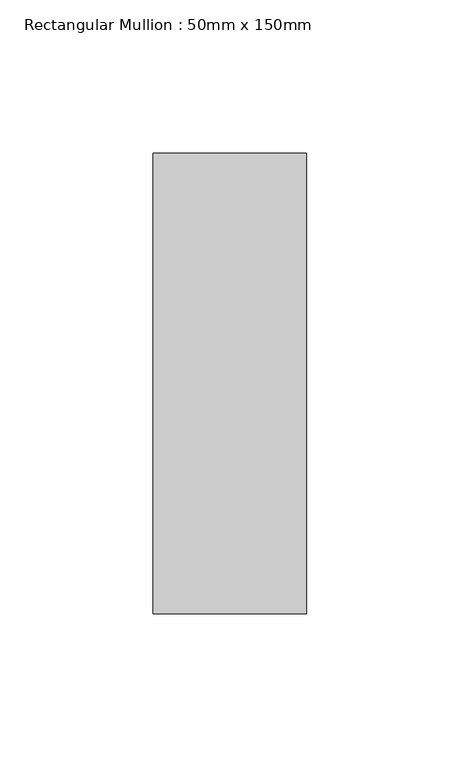
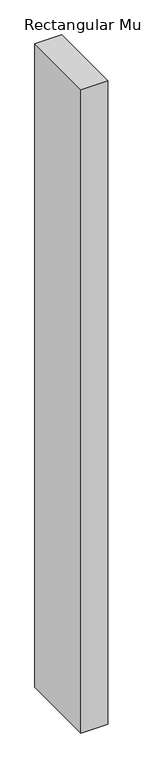
"""IFC4 building model written with IfcOpenShell, lengths in millimetres: member geometry, Rectangular Mullion : 50mm x 150mm."""

from ifc_helpers import new_model, si_unit, frame, origin, place, context, project, spatial, polyline, outline, extrude, source, transform, mapped, element, save


def rectangular_mullion_50mm_x_150mm_f38f42f6(model_context):
    return source(origin(), model_context, "Body", "SweptSolid", [
        extrude(outline(polyline([(25.0, 75.0), (25.0, -75.0), (-25.0, -75.0), (-25.0, 75.0), (25.0, 75.0)])), frame((0.0, 0.0, -1278.5714285), z_axis=(0.0, 0.0, 1.0), x_axis=(1.0, 0.0, 0.0)), (0.0, 0.0, 1.0), 1278.5714285),
    ])


if __name__ == "__main__":
    model = new_model("IFC4")
    model_context = context("Model", 3, world=origin())
    ifc_project = project(units=[si_unit("LENGTHUNIT", "METRE", prefix="MILLI")], contexts=[model_context])
    site = spatial("IfcSite", under=ifc_project)
    building = spatial("IfcBuilding", under=site)
    placement = place(None, origin())
    rectangular_mullion_50mm_x_150mm_shape = rectangular_mullion_50mm_x_150mm_f38f42f6(model_context)
    element("IfcMember", 1, ObjectType="Rectangular Mullion : 50mm x 150mm", at=placement, inside=building, context=model_context, shape_type="MappedRepresentation", body=[
        mapped(rectangular_mullion_50mm_x_150mm_shape, transform((0.0, 0.0, 0.0), x_axis=(1.0, 0.0, 0.0), y_axis=(0.0, 1.0, 0.0), z_axis=(0.0, 0.0, 1.0))),
    ])
    save(model, "model.ifc")

# Revit data of these elements
# Type "Rectangular Mullion : 50mm x 150mm"
#   built-in parameter 1007304 = 0.492126 (stored number, unit not read)
#   built-in parameter 1007301 = 0.082021 (stored number, unit not read)
#   built-in parameter 1007300 = 0.082021 (stored number, unit not read)
# Element 1 (IfcMember, "Rectangular Mullion : 50mm x 150mm")
#   Materials on its faces: "Aluminum"
# Materials
#   "Aluminum": class "Metal", colour RGB 247 247 247, transparency 0, Description = "Aluminum 6061", Cost = 0
